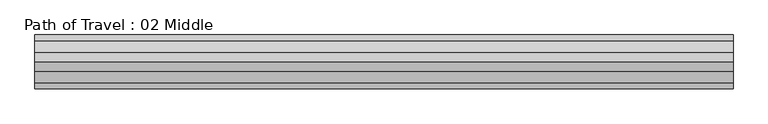
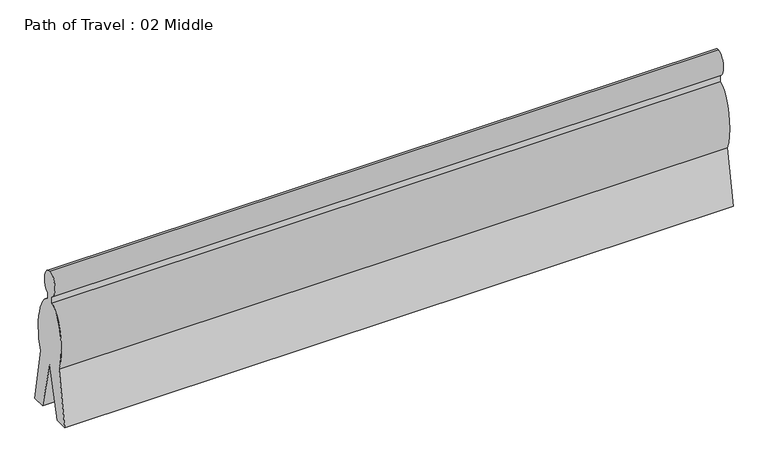
"""IFC4 building model written with IfcOpenShell, lengths in millimetres: proxy geometry, Path of Travel : 02 Middle."""

from ifc_helpers import new_model, si_unit, point, frame, origin, place, context, project, spatial, ellipse_curve, trimmed, source, transform, mapped, element, save
from ifc_brep_helpers import plane_surface, extruded_surface, advanced_brep


def path_of_travel_02_middle_7ea43315(model_context):
    return source(origin(), model_context, "Body", "AdvancedBrep", [
        advanced_brep(
        [(227.5554837, 0.0, 1727.2), (227.5554837, 42.9018657, 1436.6534209), (227.5554837, 42.9018657, 1363.4763406), (227.5554837, 184.1186263, 643.4144547), (227.5554837, 297.5699544, 0.0), (227.5554837, 145.6574193, 0.0), (227.5554837, 0.0, 584.2), (227.5554837, -145.6574193, 0.0), (227.5554837, -297.5699544, 0.0), (227.5554837, -184.1186263, 643.4144547), (227.5554837, -42.9018657, 1363.4763406), (227.5554837, -42.9018657, 1436.6534209), (7927.7574914, 0.0, 1727.2), (7927.7574914, -42.9018657, 1436.6534209), (7927.7574914, -42.9018657, 1363.4763406), (7927.7574914, -184.1186263, 643.4144547), (7927.7574914, -297.5699544, 0.0), (7927.7574914, -145.6574193, 0.0), (7927.7574914, 0.0, 584.2), (7927.7574914, 145.6574193, 0.0), (7927.7574914, 297.5699544, 0.0), (7927.7574914, 184.1186263, 643.4144547), (7927.7574914, 42.9018657, 1363.4763406), (7927.7574914, 42.9018657, 1436.6534209)],
        [
            (0, 1, ellipse_curve(frame((227.5554837, 0.0, 1574.8), z_axis=(-1.0, 0.0, 0.0), x_axis=(0.0, 0.0, 1.0)), 152.4, 101.6)),
            (1, 2),
            (2, 3, ellipse_curve(frame((227.5554837, 0.0, 914.4), z_axis=(-1.0, 0.0, 0.0), x_axis=(0.0, 0.0, -1.0)), 457.2, 228.6)),
            (3, 4),
            (4, 5),
            (5, 6),
            (6, 7),
            (7, 8),
            (8, 9),
            (9, 10, ellipse_curve(frame((227.5554837, 0.0, 914.4), z_axis=(-1.0, 0.0, 0.0), x_axis=(0.0, 0.0, -1.0)), 457.2, 228.6)),
            (10, 11),
            (11, 0, ellipse_curve(frame((227.5554837, 0.0, 1574.8), z_axis=(-1.0, 0.0, 0.0), x_axis=(0.0, 0.0, 1.0)), 152.4, 101.6)),
            (12, 13, ellipse_curve(frame((7927.7574914, 0.0, 1574.8), z_axis=(1.0, 0.0, 0.0), x_axis=(0.0, 0.0, 1.0)), 152.4, 101.6)),
            (13, 14),
            (14, 15, ellipse_curve(frame((7927.7574914, 0.0, 914.4), z_axis=(1.0, 0.0, 0.0), x_axis=(0.0, 0.0, -1.0)), 457.2, 228.6)),
            (15, 16),
            (16, 17),
            (17, 18),
            (18, 19),
            (19, 20),
            (20, 21),
            (21, 22, ellipse_curve(frame((7927.7574914, 0.0, 914.4), z_axis=(1.0, 0.0, 0.0), x_axis=(0.0, 0.0, -1.0)), 457.2, 228.6)),
            (22, 23),
            (23, 12, ellipse_curve(frame((7927.7574914, 0.0, 1574.8), z_axis=(1.0, 0.0, 0.0), x_axis=(0.0, 0.0, 1.0)), 152.4, 101.6)),
            (0, 12),
            (23, 1),
            (22, 2),
            (21, 3),
            (20, 4),
            (19, 5),
            (18, 6),
            (17, 7),
            (16, 8),
            (15, 9),
            (14, 10),
            (13, 11),
        ],
        [
            plane_surface(frame((227.5554837, 0.0, 0.0), z_axis=(-1.0, 0.0, 0.0), x_axis=(0.0, 0.0, 1.0))),
            plane_surface(frame((7927.7574914, 0.0, 0.0), z_axis=(1.0, 0.0, 0.0), x_axis=(0.0, 0.0, 1.0))),
            extruded_surface(trimmed(ellipse_curve(frame((7927.7574914, 0.0, 1574.8), z_axis=(-1.0, 0.0, 0.0), x_axis=(0.0, 0.0, 1.0)), 152.4, 101.6), [point((7927.7574914, 0.0, 1727.2))], [point((7927.7574914, 42.9018657, 1436.6534209))], True, "CARTESIAN"), (-7700.2020077, 0.0, 0.0), 7700.2020077),
            plane_surface(frame((227.5554837, 42.9018657, 1436.6534209), z_axis=(0.0, 1.0, 0.0), x_axis=(1.0, 0.0, 0.0))),
            extruded_surface(trimmed(ellipse_curve(frame((7927.7574914, 0.0, 914.4), z_axis=(-1.0, 0.0, 0.0), x_axis=(0.0, 0.0, -1.0)), 457.2, 228.6), [point((7927.7574914, 42.9018657, 1363.4763406))], [point((7927.7574914, 184.1186263, 643.4144547))], True, "CARTESIAN"), (-7700.2020077, 0.0, 0.0), 7700.2020077),
            plane_surface(frame((227.5554837, 184.1186263, 643.4144547), z_axis=(0.0, 0.9848077530122078, 0.17364817766693205), x_axis=(1.0, 0.0, 0.0))),
            plane_surface(frame((227.5554837, 297.5699544, 0.0), z_axis=(0.0, 0.0, -1.0), x_axis=(1.0, 0.0, 0.0))),
            plane_surface(frame((227.5554837, 145.6574193, 0.0), z_axis=(0.0, -0.9702957262760199, -0.2419218955995739), x_axis=(1.0, 0.0, 0.0))),
            plane_surface(frame((227.5554837, 0.0, 584.2), z_axis=(0.0, 0.9702957262759961, -0.24192189559966923), x_axis=(1.0, 0.0, 0.0))),
            plane_surface(frame((227.5554837, -145.6574193, 0.0), z_axis=(0.0, 0.0, -1.0), x_axis=(1.0, 0.0, 0.0))),
            plane_surface(frame((227.5554837, -297.5699544, 0.0), z_axis=(0.0, -0.984807753012208, 0.17364817766693066), x_axis=(1.0, 0.0, 0.0))),
            extruded_surface(trimmed(ellipse_curve(frame((7927.7574914, 0.0, 914.4), z_axis=(-1.0, 0.0, 0.0), x_axis=(0.0, 0.0, -1.0)), 457.2, 228.6), [point((7927.7574914, -184.1186263, 643.4144547))], [point((7927.7574914, -42.9018657, 1363.4763406))], True, "CARTESIAN"), (-7700.2020077, 0.0, 0.0), 7700.2020077),
            plane_surface(frame((227.5554837, -42.9018657, 1363.4763406), z_axis=(0.0, -1.0, 0.0), x_axis=(1.0, 0.0, 0.0))),
            extruded_surface(trimmed(ellipse_curve(frame((7927.7574914, 0.0, 1574.8), z_axis=(-1.0, 0.0, 0.0), x_axis=(0.0, 0.0, 1.0)), 152.4, 101.6), [point((7927.7574914, -42.9018657, 1436.6534209))], [point((7927.7574914, 0.0, 1727.2))], True, "CARTESIAN"), (-7700.2020077, 0.0, 0.0), 7700.2020077),
        ],
        [
            (0, [[1, 2, 3, 4, 5, 6, 7, 8, 9, 10, 11, 12]]),
            (1, [[13, 14, 15, 16, 17, 18, 19, 20, 21, 22, 23, 24]]),
            (2, [[-1, 25, -24, 26]]),
            (3, [[-2, -26, -23, 27]]),
            (4, [[-3, -27, -22, 28]]),
            (5, [[-4, -28, -21, 29]]),
            (6, [[-5, -29, -20, 30]]),
            (7, [[-6, -30, -19, 31]]),
            (8, [[-7, -31, -18, 32]]),
            (9, [[-8, -32, -17, 33]]),
            (10, [[-9, -33, -16, 34]]),
            (11, [[-10, -34, -15, 35]]),
            (12, [[-11, -35, -14, 36]]),
            (13, [[-12, -36, -13, -25]]),
        ],
    ),
    ])


if __name__ == "__main__":
    model = new_model("IFC4")
    model_context = context("Model", 3, world=origin())
    ifc_project = project(units=[si_unit("LENGTHUNIT", "METRE", prefix="MILLI")], contexts=[model_context])
    site = spatial("IfcSite", under=ifc_project)
    building = spatial("IfcBuilding", under=site)
    placement = place(None, origin())
    path_of_travel_02_middle_shape = path_of_travel_02_middle_7ea43315(model_context)
    element("IfcBuildingElementProxy", 1, Name="Path of Travel : 02 Middle", ObjectType="Path of Travel : 02 Middle", at=placement, inside=building, context=model_context, shape_type="MappedRepresentation", body=[
        mapped(path_of_travel_02_middle_shape, transform((0.0, 0.0, 0.0), x_axis=(1.0, 0.0, 0.0), y_axis=(0.0, 1.0, 0.0), z_axis=(0.0, 0.0, 1.0))),
    ])
    save(model, "model.ifc")

# Revit data of these elements
# Type "Path of Travel : 02 Middle"
#   Path of Egress [instance default] = 4' - 0"
#   built-in parameter 1001306 [instance default] = 4 (stored number, unit not read)
#   Dot at Start = no
#   Arrow in Middle = yes
#   Arrow at End = no
#   Egress Path = none
# Element 1 (IfcBuildingElementProxy, "Path of Travel : 02 Middle")
#   Path of Egress = 25' - 3.15756"
#   built-in parameter 1001306 = 25.2631 (stored number, unit not read)
#   Materials on its faces: "Egress Path Solid"
# Materials
#   "Egress Path Solid": class "Unassigned", colour RGB 255 128 64, transparency 0.75, Comments = "Rendering appearance not upgraded "
